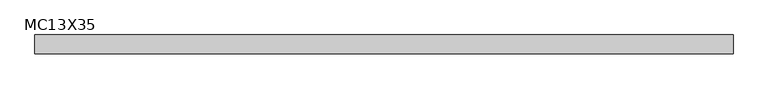
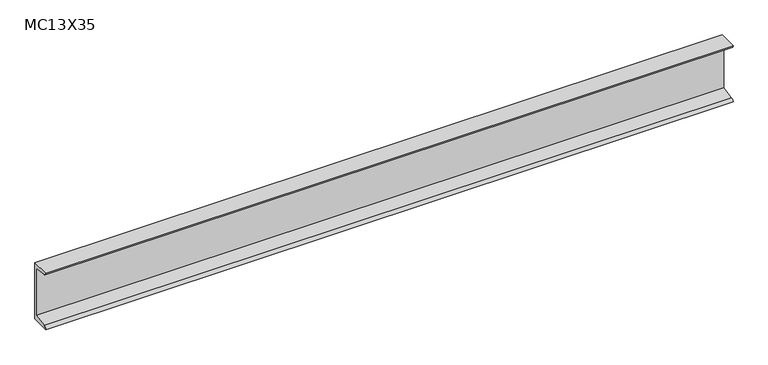
"""IFC4 building model written with IfcOpenShell, lengths in millimetres: beam geometry, MC-Miscellaneous Channel : MC13X35."""

from ifc_helpers import new_model, si_unit, point, frame, frame_2d, origin, place, context, project, spatial, polyline, circle_curve, trimmed, segment, composite_curve, outline, extrude, source, transform, mapped, element, save


def mc13x35_ea4ffe94(model_context):
    return source(origin(), model_context, "Body", "SweptSolid", [
        extrude(outline(composite_curve([segment(polyline([(24.892, 165.1), (24.892, -165.1), (-78.486, -165.1)]), True, "CONTINUOUS"), segment(trimmed(circle_curve(frame_2d((-62.992, -165.1)), 15.494), [point((-78.486, -165.1))], [point((-62.992, -149.606))], False, "CARTESIAN"), True, "CONTINUOUS"), segment(polyline([(-62.992, -149.606), (13.5382, -137.4848071), (13.5382, 137.4848071), (-62.992, 149.606)]), True, "CONTINUOUS"), segment(trimmed(circle_curve(frame_2d((-62.992, 165.1)), 15.494), [point((-62.992, 149.606))], [point((-78.486, 165.1))], False, "CARTESIAN"), True, "CONTINUOUS"), segment(polyline([(-78.486, 165.1), (24.892, 165.1)]), True, "CONTINUOUS")], self_intersect=False)), frame((-1917.7, 0.0, 0.0), z_axis=(1.0, 0.0, 0.0), x_axis=(0.0, 1.0, 0.0)), (0.0, 0.0, 1.0), 3810.0),
    ])


if __name__ == "__main__":
    model = new_model("IFC4")
    model_context = context("Model", 3, world=origin())
    ifc_project = project(units=[si_unit("LENGTHUNIT", "METRE", prefix="MILLI")], contexts=[model_context])
    site = spatial("IfcSite", under=ifc_project)
    building = spatial("IfcBuilding", under=site)
    placement = place(None, origin())
    mc13x35_shape = mc13x35_ea4ffe94(model_context)
    element("IfcBeam", 1, ObjectType="MC-Miscellaneous Channel : MC13X35", at=placement, inside=building, context=model_context, shape_type="MappedRepresentation", body=[
        mapped(mc13x35_shape, transform((0.0, 0.0, 0.0), x_axis=(1.0, 0.0, 0.0), y_axis=(0.0, 1.0, 0.0), z_axis=(0.0, 0.0, 1.0))),
    ])
    save(model, "model.ifc")

# Revit data of these elements
# Type "MC-Miscellaneous Channel : MC13X35"
#   Assembly Code = "B10"
#   W = 35
#   Length [instance default] = 5' - 0"
#   bf = 0' - 4.07"
#   d = 1' - 1"
#   tf = 0' - 0.61"
#   tw = 0' - 0.447"
#   x = 0' - 0.98"
#   A = 0.0715278 SF
#   Structural Material [instance default] = Steel ASTM A36
# Element 1 (IfcBeam, "MC-Miscellaneous Channel : MC13X35")
#   Structural Material = Steel ASTM A992
#   Materials on its faces: "Steel ASTM A992"
# Materials
#   "Steel ASTM A36": class "Metal", colour RGB 199 199 199, transparency 0, Description = "Structural steel, ASTM A36 Grade B, mill finish", Cost = 0
#   "Steel ASTM A992": class "Metal", colour RGB 199 199 199, transparency 0, Description = "Structural steel 50ksi", Cost = 0
